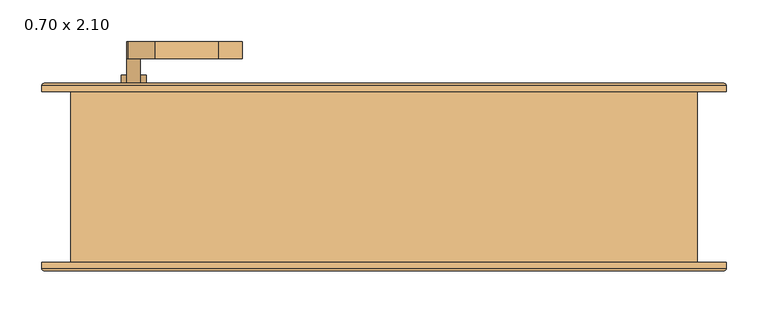
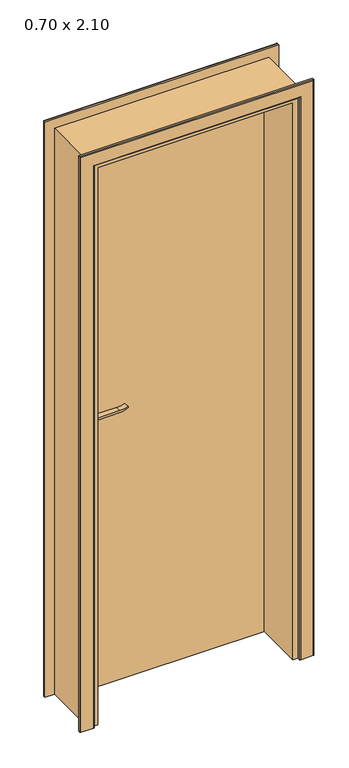
"""IFC4 building model written with IfcOpenShell, lengths in millimetres: door geometry, .CC_ND 300_PORTA SIMPLES DE ABRIR_COM EXTENSÃO : 0.70 x 2.10."""

from ifc_helpers import new_model, si_unit, point, frame, frame_2d, origin, origin_with_axes, place, context, project, spatial, polyline, circle_curve, ellipse_curve, trimmed, segment, composite_curve, outline, extrude, faceted_brep, source, transform, mapped, element, save
from ifc_brep_helpers import plane_surface, cylinder_surface, advanced_brep


def door_0_70_x_2_10_c4bac616(model_context):
    return source(origin(), model_context, "Body", "SolidModel", [
        extrude(outline(composite_curve([segment(trimmed(circle_curve(frame_2d((964.5, -300.0)), 15.0), [point((964.5, -285.0))], [point((964.5, -315.0))], False, "CARTESIAN"), True, "CONTINUOUS"), segment(trimmed(circle_curve(frame_2d((964.5, -300.0)), 15.0), [point((964.5, -315.0))], [point((964.5, -285.0))], False, "CARTESIAN"), True, "CONTINUOUS")], self_intersect=False)), frame((0.0, 127.9, 0.0), z_axis=(0.0, 1.0, 0.0), x_axis=(0.0, 0.0, 1.0)), (0.0, 0.0, 1.0), 10.0),
        extrude(outline(composite_curve([segment(trimmed(circle_curve(frame_2d((964.5, -300.0)), 15.0), [point((964.5, -285.0))], [point((964.5, -315.0))], False, "CARTESIAN"), True, "CONTINUOUS"), segment(trimmed(circle_curve(frame_2d((964.5, -300.0)), 15.0), [point((964.5, -315.0))], [point((964.5, -285.0))], False, "CARTESIAN"), True, "CONTINUOUS")], self_intersect=False)), frame((0.0, 67.9, 0.0), z_axis=(0.0, 1.0, 0.0), x_axis=(0.0, 0.0, 1.0)), (0.0, 0.0, 1.0), 10.0),
        extrude(outline(composite_curve([segment(trimmed(circle_curve(frame_2d((1024.5, -300.0)), 8.0), [point((1029.1523287, -306.5081363))], [point((1024.5, -292.0))], False, "CARTESIAN"), True, "CONTINUOUS"), segment(trimmed(circle_curve(frame_2d((1019.3738613, -274.6138099)), 18.1261387), [point((1024.5, -292.0))], [point((1037.5, -274.6138099))], True, "CARTESIAN"), True, "CONTINUOUS"), segment(polyline([(1037.5, -274.6138099), (1037.5, -198.3564091)]), True, "CONTINUOUS"), segment(trimmed(circle_curve(frame_2d((1096.7709207, -201.9396612)), 59.3791355), [point((1037.5, -198.3564091))], [point((1046.7135558, -170.0))], False, "CARTESIAN"), True, "CONTINUOUS"), segment(polyline([(1046.7135558, -170.0), (1049.5, -170.0)]), True, "CONTINUOUS"), segment(trimmed(circle_curve(frame_2d((1127.7850638, -198.4227909)), 83.2850902), [point((1049.5, -170.0))], [point((1044.5, -198.3564091))], True, "CARTESIAN"), True, "CONTINUOUS"), segment(polyline([(1044.5, -198.3564091), (1044.5, -274.6325667)]), True, "CONTINUOUS"), segment(trimmed(circle_curve(frame_2d((1007.2555521, -276.3324871)), 37.2832219), [point((1044.5, -274.6325667))], [point((1029.1523287, -306.5081363))], False, "CARTESIAN"), True, "CONTINUOUS")], self_intersect=False)), frame((0.0, 157.9, 0.0), z_axis=(0.0, 1.0, 0.0), x_axis=(0.0, 0.0, 1.0)), (0.0, 0.0, 1.0), 20.0),
        extrude(outline(composite_curve([segment(trimmed(circle_curve(frame_2d((1019.3738682, -274.6138122)), 18.1261318), [point((1024.4999903, -292.0))], [point((1037.5, -274.6138122))], True, "CARTESIAN"), True, "CONTINUOUS"), segment(polyline([(1037.5, -274.6138122), (1037.5, -198.3564091)]), True, "CONTINUOUS"), segment(trimmed(circle_curve(frame_2d((1096.7709207, -201.9396612)), 59.3791355), [point((1037.5, -198.3564091))], [point((1046.7135558, -170.0))], False, "CARTESIAN"), True, "CONTINUOUS"), segment(polyline([(1046.7135558, -170.0), (1049.5, -170.0)]), True, "CONTINUOUS"), segment(trimmed(circle_curve(frame_2d((1127.7850638, -198.4227909)), 83.2850902), [point((1049.5, -170.0))], [point((1044.5, -198.3564091))], True, "CARTESIAN"), True, "CONTINUOUS"), segment(polyline([(1044.5, -198.3564091), (1044.5, -274.6325667)]), True, "CONTINUOUS"), segment(trimmed(circle_curve(frame_2d((1007.2555521, -276.3324871)), 37.2832219), [point((1044.5, -274.6325667))], [point((1029.1523287, -306.5081363))], False, "CARTESIAN"), True, "CONTINUOUS"), segment(trimmed(circle_curve(frame_2d((1024.5, -300.0)), 8.0), [point((1029.1523287, -306.5081363))], [point((1024.4999903, -292.0))], False, "CARTESIAN"), True, "CONTINUOUS")], self_intersect=False)), frame((0.0, 27.9, 0.0), z_axis=(0.0, 1.0, 0.0), x_axis=(0.0, 0.0, 1.0)), (0.0, 0.0, 1.0), 20.0),
        extrude(outline(composite_curve([segment(trimmed(circle_curve(frame_2d((1024.5, -300.0)), 8.0), [point((1024.5, -292.0))], [point((1024.5, -308.0))], False, "CARTESIAN"), True, "CONTINUOUS"), segment(trimmed(circle_curve(frame_2d((1024.5, -300.0)), 8.0), [point((1024.5, -308.0))], [point((1024.5, -292.0))], False, "CARTESIAN"), True, "CONTINUOUS")], self_intersect=False)), frame((0.0, 127.9, 0.0), z_axis=(0.0, 1.0, 0.0), x_axis=(0.0, 0.0, 1.0)), (0.0, 0.0, 1.0), 30.0),
        extrude(outline(composite_curve([segment(trimmed(circle_curve(frame_2d((1024.5, -300.0)), 8.0), [point((1024.5, -292.0))], [point((1024.5, -308.0))], False, "CARTESIAN"), True, "CONTINUOUS"), segment(trimmed(circle_curve(frame_2d((1024.5, -300.0)), 8.0), [point((1024.5, -308.0))], [point((1024.5, -292.0))], False, "CARTESIAN"), True, "CONTINUOUS")], self_intersect=False)), frame((0.0, 47.9, 0.0), z_axis=(0.0, 1.0, 0.0), x_axis=(0.0, 0.0, 1.0)), (0.0, 0.0, 1.0), 30.0),
        extrude(outline(composite_curve([segment(trimmed(circle_curve(frame_2d((954.5, -300.0)), 25.0), [point((954.5, -325.0))], [point((954.5, -275.0))], False, "CARTESIAN"), True, "CONTINUOUS"), segment(polyline([(954.5, -275.0), (1024.5, -275.0)]), True, "CONTINUOUS"), segment(trimmed(circle_curve(frame_2d((1024.5, -300.0)), 25.0), [point((1024.5, -275.0))], [point((1024.5, -325.0))], False, "CARTESIAN"), True, "CONTINUOUS"), segment(polyline([(1024.5, -325.0), (954.5, -325.0)]), True, "CONTINUOUS")], self_intersect=False)), frame((0.0, 117.9, 0.0), z_axis=(0.0, 1.0, 0.0), x_axis=(0.0, 0.0, 1.0)), (0.0, 0.0, 1.0), 10.0),
        extrude(outline(composite_curve([segment(trimmed(circle_curve(frame_2d((954.5, -300.0)), 25.0), [point((954.5, -325.0))], [point((954.5, -275.0))], False, "CARTESIAN"), True, "CONTINUOUS"), segment(polyline([(954.5, -275.0), (1024.5, -275.0)]), True, "CONTINUOUS"), segment(trimmed(circle_curve(frame_2d((1024.5, -300.0)), 25.0), [point((1024.5, -275.0))], [point((1024.5, -325.0))], False, "CARTESIAN"), True, "CONTINUOUS"), segment(polyline([(1024.5, -325.0), (954.5, -325.0)]), True, "CONTINUOUS")], self_intersect=False)), frame((0.0, 77.9, 0.0), z_axis=(0.0, 1.0, 0.0), x_axis=(0.0, 0.0, 1.0)), (0.0, 0.0, 1.0), 10.0),
        faceted_brep([(342.0, -86.9, 0.0), (342.0, 87.9, 0.0), (350.0, 87.9, 0.0), (350.0, 117.9, 0.0), (375.0, 117.9, 0.0), (375.0, -86.9, 0.0), (375.0, -86.9, 2100.0), (-375.0, -86.9, 2100.0), (-375.0, -86.9, 0.0), (-342.0, -86.9, 0.0), (-342.0, -86.9, 2067.0), (342.0, -86.9, 2067.0), (375.0, 117.9, 2100.0), (350.0, 117.9, 2075.0), (-350.0, 117.9, 2075.0), (-350.0, 117.9, 0.0), (-375.0, 117.9, 0.0), (-375.0, 117.9, 2100.0), (350.0, 87.9, 2075.0), (342.0, 87.9, 2067.0), (-342.0, 87.9, 2067.0), (-342.0, 87.9, 0.0), (-350.0, 87.9, 0.0), (-350.0, 87.9, 2075.0)], [[[0, 1, 2, 3, 4, 5]], [[5, 6, 7, 8, 9, 10, 11, 0]], [[4, 12, 6, 5]], [[3, 13, 14, 15, 16, 17, 12, 4]], [[2, 18, 13, 3]], [[1, 19, 20, 21, 22, 23, 18, 2]], [[0, 11, 19, 1]], [[10, 9, 21, 20]], [[9, 8, 16, 15, 22, 21]], [[17, 16, 8, 7]], [[23, 22, 15, 14]], [[12, 17, 7, 6]], [[18, 23, 14, 13]], [[11, 10, 20, 19]]]),
        extrude(outline(polyline([(-350.0, 87.9), (-350.0, 117.9), (350.0, 117.9), (350.0, 87.9), (-350.0, 87.9)])), origin_with_axes(), (0.0, 0.0, 1.0), 2075.0),
        advanced_brep(
        [(-410.0, 117.9, 0.0), (-410.0, 124.9, 0.0), (-407.0, 127.9, 0.0), (-363.0, 127.9, 0.0), (-360.0, 124.9, 0.0), (-360.0, 117.9, 0.0), (-360.0, 117.9, 2085.0), (360.0, 117.9, 2085.0), (360.0, 117.9, 0.0), (410.0, 117.9, 0.0), (410.0, 117.9, 2135.0), (-410.0, 117.9, 2135.0), (-360.0, 124.9, 2085.0), (-363.0, 127.9, 2088.0), (-407.0, 127.9, 2132.0), (407.0, 127.9, 2132.0), (407.0, 127.9, 0.0), (363.0, 127.9, 0.0), (363.0, 127.9, 2088.0), (-410.0, 124.9, 2135.0), (410.0, 124.9, 0.0), (410.0, 124.9, 2135.0), (360.0, 124.9, 0.0), (360.0, 124.9, 2085.0)],
        [
            (0, 1),
            (1, 2, circle_curve(frame((-407.0, 124.9, 0.0), z_axis=(0.0, 0.0, -1.0), x_axis=(1.0, 0.0, 0.0)), 3.0)),
            (2, 3),
            (3, 4, circle_curve(frame((-363.0, 124.9, 0.0), z_axis=(0.0, 0.0, -1.0), x_axis=(1.0, 0.0, 0.0)), 3.0)),
            (4, 5),
            (5, 0),
            (5, 6),
            (6, 7),
            (7, 8),
            (8, 9),
            (9, 10),
            (10, 11),
            (11, 0),
            (4, 12),
            (12, 6),
            (3, 13),
            (13, 12, ellipse_curve(frame((-363.0, 124.9, 2088.0), z_axis=(-0.7071067811865475, 0.0, -0.7071067811865475), x_axis=(0.7071067811865474, 0.0, -0.7071067811865476)), 4.2426407, 3.0)),
            (2, 14),
            (14, 15),
            (15, 16),
            (16, 17),
            (17, 18),
            (18, 13),
            (1, 19),
            (19, 14, ellipse_curve(frame((-407.0, 124.9, 2132.0), z_axis=(-0.7071067811865475, 0.0, -0.7071067811865475), x_axis=(0.7071067811865474, 0.0, -0.7071067811865476)), 4.2426407, 3.0)),
            (11, 19),
            (9, 20),
            (20, 21),
            (21, 10),
            (8, 22),
            (22, 17, circle_curve(frame((363.0, 124.9, 0.0), z_axis=(0.0, 0.0, -1.0), x_axis=(-1.0, 0.0, 0.0)), 3.0)),
            (16, 20, circle_curve(frame((407.0, 124.9, 0.0), z_axis=(0.0, 0.0, -1.0), x_axis=(-1.0, 0.0, 0.0)), 3.0)),
            (23, 22),
            (7, 23),
            (23, 18, ellipse_curve(frame((363.0, 124.9, 2088.0), z_axis=(0.7071067811865475, 0.0, -0.7071067811865475), x_axis=(0.7071067811865474, 0.0, 0.7071067811865476)), 4.2426407, 3.0)),
            (15, 21, ellipse_curve(frame((407.0, 124.9, 2132.0), z_axis=(0.7071067811865475, 0.0, -0.7071067811865475), x_axis=(0.7071067811865474, 0.0, 0.7071067811865476)), 4.2426407, 3.0)),
            (12, 23),
            (21, 19),
        ],
        [
            plane_surface(frame((-360.0, 117.9, 0.0), z_axis=(0.0, 0.0, -1.0), x_axis=(0.0, -1.0, 0.0))),
            plane_surface(frame((-410.0, 117.9, 0.0), z_axis=(0.0, -1.0, 0.0), x_axis=(0.0, 0.0, 1.0))),
            plane_surface(frame((-360.0, 117.9, 0.0), z_axis=(1.0, 0.0, 0.0), x_axis=(0.0, 0.0, 1.0))),
            cylinder_surface(frame((-363.0, 124.9, 0.0), z_axis=(0.0, 0.0, -1.0), x_axis=(1.0, 0.0, 0.0)), 3.0),
            plane_surface(frame((-363.0, 127.9, 0.0), z_axis=(0.0, 1.0, 0.0), x_axis=(0.0, 0.0, 1.0))),
            cylinder_surface(frame((-407.0, 124.9, 0.0), z_axis=(0.0, 0.0, -1.0), x_axis=(1.0, 0.0, 0.0)), 3.0),
            plane_surface(frame((-410.0, 124.9, 0.0), z_axis=(-1.0, 0.0, 0.0), x_axis=(0.0, 0.0, 1.0))),
            plane_surface(frame((410.0, 124.9, 2135.0), z_axis=(1.0, 0.0, 0.0), x_axis=(0.0, 0.0, -1.0))),
            plane_surface(frame((360.0, 117.9, 0.0), z_axis=(0.0, 0.0, -1.0), x_axis=(0.0, -1.0, 0.0))),
            plane_surface(frame((360.0, 117.9, 2085.0), z_axis=(-1.0, 0.0, 0.0), x_axis=(0.0, 0.0, -1.0))),
            cylinder_surface(frame((363.0, 124.9, 2085.0), z_axis=(0.0, 0.0, 1.0), x_axis=(-1.0, 0.0, 0.0)), 3.0),
            cylinder_surface(frame((407.0, 124.9, 2085.0), z_axis=(0.0, 0.0, 1.0), x_axis=(-1.0, 0.0, 0.0)), 3.0),
            plane_surface(frame((-360.0, 117.9, 2085.0), z_axis=(0.0, 0.0, -1.0), x_axis=(1.0, 0.0, 0.0))),
            plane_surface(frame((-410.0, 124.9, 2135.0), z_axis=(0.0, 0.0, 1.0), x_axis=(1.0, 0.0, 0.0))),
            cylinder_surface(frame((-360.0, 124.9, 2088.0), z_axis=(-1.0, 0.0, 0.0), x_axis=(0.0, 0.0, -1.0)), 3.0),
            cylinder_surface(frame((-360.0, 124.9, 2132.0), z_axis=(-1.0, 0.0, 0.0), x_axis=(0.0, 0.0, -1.0)), 3.0),
        ],
        [
            (0, [[1, 2, 3, 4, 5, 6]]),
            (1, [[7, 8, 9, 10, 11, 12, 13, -6]]),
            (2, [[14, 15, -7, -5]]),
            (3, [[16, 17, -14, -4]]),
            (4, [[18, 19, 20, 21, 22, 23, -16, -3]]),
            (5, [[24, 25, -18, -2]]),
            (6, [[-13, 26, -24, -1]]),
            (7, [[-11, 27, 28, 29]]),
            (8, [[-10, 30, 31, -21, 32, -27]]),
            (9, [[33, -30, -9, 34]]),
            (10, [[-22, -31, -33, 35]]),
            (11, [[-28, -32, -20, 36]]),
            (12, [[37, -34, -8, -15]]),
            (13, [[-12, -29, 38, -26]]),
            (14, [[-23, -35, -37, -17]]),
            (15, [[-38, -36, -19, -25]]),
        ],
    ),
        advanced_brep(
        [(410.0, -86.9, 0.0), (410.0, -93.9342217, 0.0), (407.0342217, -96.9, 0.0), (362.9842717, -96.9, 0.0), (360.0, -93.9157283, 0.0), (360.0, -86.9, 0.0), (360.0, -86.9, 2085.0), (-360.0, -86.9, 2085.0), (-360.0, -86.9, 0.0), (-410.0, -86.9, 0.0), (-410.0, -86.9, 2135.0), (410.0, -86.9, 2135.0), (360.0, -93.9157283, 2085.0), (362.9842717, -96.9, 2087.9842717), (407.0342217, -96.9, 2132.0342217), (-407.0342217, -96.9, 2132.0342217), (-407.0342217, -96.9, 0.0), (-362.9842717, -96.9, 0.0), (-362.9842717, -96.9, 2087.9842717), (410.0, -93.9342217, 2135.0), (-410.0, -93.9342217, 0.0), (-410.0, -93.9342217, 2135.0), (-360.0, -93.9157283, 0.0), (-360.0, -93.9157283, 2085.0)],
        [
            (0, 1),
            (1, 2, circle_curve(frame((407.0342217, -93.9342217, 0.0), z_axis=(0.0, 0.0, -1.0), x_axis=(1.0, 0.0, 0.0)), 2.9657783)),
            (2, 3),
            (3, 4, circle_curve(frame((362.9842717, -93.9157283, 0.0), z_axis=(0.0, 0.0, -1.0), x_axis=(1.0, 0.0, 0.0)), 2.9842717)),
            (4, 5),
            (5, 0),
            (5, 6),
            (6, 7),
            (7, 8),
            (8, 9),
            (9, 10),
            (10, 11),
            (11, 0),
            (4, 12),
            (12, 6),
            (3, 13),
            (13, 12, ellipse_curve(frame((362.9842717, -93.9157283, 2087.9842717), z_axis=(0.7071067811865475, 0.0, -0.7071067811865475), x_axis=(-0.7071067811865474, 0.0, -0.7071067811865476)), 4.2203975, 2.9842717)),
            (2, 14),
            (14, 15),
            (15, 16),
            (16, 17),
            (17, 18),
            (18, 13),
            (1, 19),
            (19, 14, ellipse_curve(frame((407.0342217, -93.9342217, 2132.0342217), z_axis=(0.7071067811865475, 0.0, -0.7071067811865475), x_axis=(-0.7071067811865474, 0.0, -0.7071067811865476)), 4.1942438, 2.9657783)),
            (11, 19),
            (9, 20),
            (20, 21),
            (21, 10),
            (8, 22),
            (22, 17, circle_curve(frame((-362.9842717, -93.9157283, 0.0), z_axis=(0.0, 0.0, -1.0), x_axis=(-1.0, 0.0, 0.0)), 2.9842717)),
            (16, 20, circle_curve(frame((-407.0342217, -93.9342217, 0.0), z_axis=(0.0, 0.0, -1.0), x_axis=(-1.0, 0.0, 0.0)), 2.9657783)),
            (23, 22),
            (7, 23),
            (23, 18, ellipse_curve(frame((-362.9842717, -93.9157283, 2087.9842717), z_axis=(-0.7071067811865475, 0.0, -0.7071067811865475), x_axis=(-0.7071067811865474, 0.0, 0.7071067811865476)), 4.2203975, 2.9842717)),
            (15, 21, ellipse_curve(frame((-407.0342217, -93.9342217, 2132.0342217), z_axis=(-0.7071067811865475, 0.0, -0.7071067811865475), x_axis=(-0.7071067811865474, 0.0, 0.7071067811865476)), 4.1942438, 2.9657783)),
            (12, 23),
            (21, 19),
        ],
        [
            plane_surface(frame((360.0, -86.9, 0.0), z_axis=(0.0, 0.0, -1.0), x_axis=(0.0, -1.0, 0.0))),
            plane_surface(frame((410.0, -86.9, 0.0), z_axis=(0.0, 1.0, 0.0), x_axis=(0.0, 0.0, 1.0))),
            plane_surface(frame((360.0, -86.9, 0.0), z_axis=(-1.0, 0.0, 0.0), x_axis=(0.0, 0.0, 1.0))),
            cylinder_surface(frame((362.9842717, -93.9157283, 0.0), z_axis=(0.0, 0.0, -1.0), x_axis=(1.0, 0.0, 0.0)), 2.9842717),
            plane_surface(frame((362.9842717, -96.9, 0.0), z_axis=(0.0, -1.0, 0.0), x_axis=(0.0, 0.0, 1.0))),
            cylinder_surface(frame((407.0342217, -93.9342217, 0.0), z_axis=(0.0, 0.0, -1.0), x_axis=(1.0, 0.0, 0.0)), 2.9657783),
            plane_surface(frame((410.0, -93.9342217, 0.0), z_axis=(1.0, 0.0, 0.0), x_axis=(0.0, 0.0, 1.0))),
            plane_surface(frame((-410.0, -93.9342217, 2135.0), z_axis=(-1.0, 0.0, 0.0), x_axis=(0.0, 0.0, -1.0))),
            plane_surface(frame((-360.0, -86.9, 0.0), z_axis=(0.0, 0.0, -1.0), x_axis=(0.0, -1.0, 0.0))),
            plane_surface(frame((-360.0, -86.9, 2085.0), z_axis=(1.0, 0.0, 0.0), x_axis=(0.0, 0.0, -1.0))),
            cylinder_surface(frame((-362.9842717, -93.9157283, 2085.0), z_axis=(0.0, 0.0, 1.0), x_axis=(-1.0, 0.0, 0.0)), 2.9842717),
            cylinder_surface(frame((-407.0342217, -93.9342217, 2085.0), z_axis=(0.0, 0.0, 1.0), x_axis=(-1.0, 0.0, 0.0)), 2.9657783),
            plane_surface(frame((360.0, -86.9, 2085.0), z_axis=(0.0, 0.0, -1.0), x_axis=(-1.0, 0.0, 0.0))),
            plane_surface(frame((410.0, -93.9342217, 2135.0), z_axis=(0.0, 0.0, 1.0), x_axis=(-1.0, 0.0, 0.0))),
            cylinder_surface(frame((360.0, -93.9157283, 2087.9842717), z_axis=(1.0, 0.0, 0.0), x_axis=(0.0, 0.0, 1.0)), 2.9842717),
            cylinder_surface(frame((360.0, -93.9342217, 2132.0342217), z_axis=(1.0, 0.0, 0.0), x_axis=(0.0, 0.0, 1.0)), 2.9657783),
        ],
        [
            (0, [[1, 2, 3, 4, 5, 6]]),
            (1, [[7, 8, 9, 10, 11, 12, 13, -6]]),
            (2, [[14, 15, -7, -5]]),
            (3, [[16, 17, -14, -4]]),
            (4, [[18, 19, 20, 21, 22, 23, -16, -3]]),
            (5, [[24, 25, -18, -2]]),
            (6, [[-13, 26, -24, -1]]),
            (7, [[-11, 27, 28, 29]]),
            (8, [[-10, 30, 31, -21, 32, -27]]),
            (9, [[33, -30, -9, 34]]),
            (10, [[-22, -31, -33, 35]]),
            (11, [[-28, -32, -20, 36]]),
            (12, [[37, -34, -8, -15]]),
            (13, [[-12, -29, 38, -26]]),
            (14, [[-23, -35, -37, -17]]),
            (15, [[-38, -36, -19, -25]]),
        ],
    ),
    ])


if __name__ == "__main__":
    model = new_model("IFC4")
    model_context = context("Model", 3, world=origin())
    ifc_project = project(units=[si_unit("LENGTHUNIT", "METRE", prefix="MILLI")], contexts=[model_context])
    site = spatial("IfcSite", under=ifc_project)
    building = spatial("IfcBuilding", under=site)
    placement = place(None, origin())
    door_0_70_x_2_10_shape = door_0_70_x_2_10_c4bac616(model_context)
    element("IfcDoor", 1, ObjectType=".CC_ND 300_PORTA SIMPLES DE ABRIR_COM EXTENSÃO : 0.70 x 2.10", at=placement, inside=building, context=model_context, shape_type="MappedRepresentation", body=[
        mapped(door_0_70_x_2_10_shape, transform((0.0, 0.0, 0.0), x_axis=(1.0, 0.0, 0.0), y_axis=(0.0, 1.0, 0.0), z_axis=(0.0, 0.0, 1.0))),
    ])
    save(model, "model.ifc")

# Revit data of these elements
# Type ".CC_ND 300_PORTA SIMPLES DE ABRIR_COM EXTENSÃO : 0.70 x 2.10"
#   Type Mark = "155"
#   Analytic Construction = "<None>"
#   Rough Width = 0.75 m
#   Espessura moldura externa = 0.01 m
#   Espessura moldura interna = 0.01 m
#   Largura moldura = 0.05 m
#   Extensão acabamento exterior [instance default] = 0.00 m
#   Extensão acabamento interior [instance default] = 0.00 m
#   Espessura batente = 0.025 m
#   Thickness = 0.03 m
#   Altura batente = 2.085 m
#   Aux Arco [instance default] = 0.70 m
#   Rough Height = 2.125 m
#   Height = 2.10 m
#   Width = 0.70 m
#   Moldura interna [instance default] = yes
#   Moldura externa [instance default] = yes
#   Porta = .MADEIRA COM PINTURA ESMALTE BRANCO ACETINADO
#   Moldura = .MADEIRA COM PINTURA ESMALTE BRANCO ACETINADO
#   Maçaneta = .ALUMÍNIO
#   Batente = .MADEIRA COM PINTURA ESMALTE BRANCO ACETINADO
#   Function = (empty or 0)
#   Wall Closure = (empty or 0)
# Element 1 (IfcDoor, ".CC_ND 300_PORTA SIMPLES DE ABRIR_COM EXTENSÃO : 0.70 x 2.10")
#   Extensão acabamento interior = 0.031 m
#   Aux Arco = 0.731 m
#   Materials on its faces: ".MADEIRA COM PINTURA ESMALTE BRANCO ACETINADO", ".ALUMÍNIO"
# Materials
#   ".MADEIRA COM PINTURA ESMALTE BRANCO ACETINADO": class ".CC_MADEIRAS", colour RGB 240 240 240, transparency 0, Description = "Madeira com pintura esmalte branco acetinado.", Cost = 0
#   ".ALUMÍNIO": class "CC_METAIS", colour RGB 244 244 244, transparency 0, Description = "Material alumínio", Cost = 0
